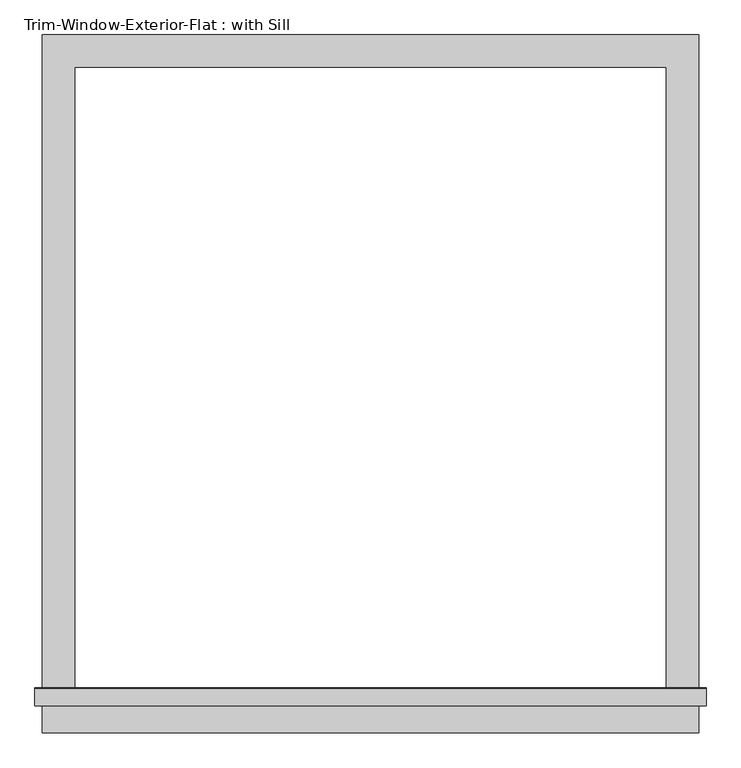
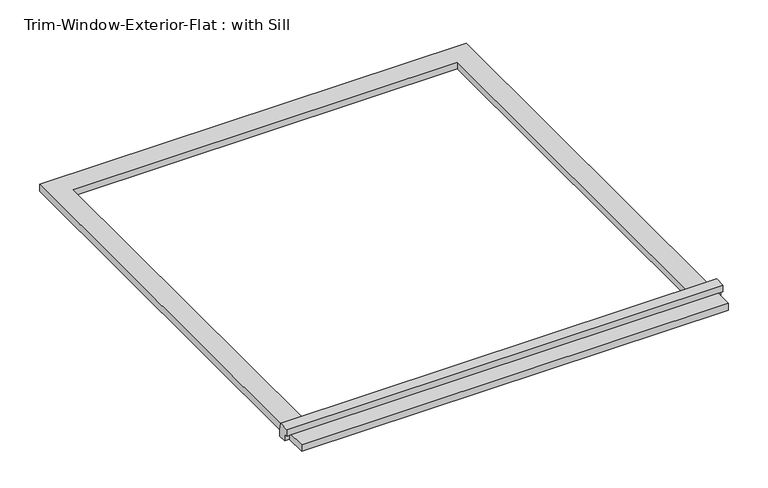
"""IFC4 building model written with IfcOpenShell, lengths in millimetres: proxy geometry, Trim-Window-Exterior-Flat : with Sill."""

import ifcopenshell
import ifcopenshell.guid

model = None  # the IFC model being written
_history = None  # IfcOwnerHistory: only IFC2X3 demands one
_inside = {}  # id of a spatial element -> (the spatial element, [elements in it])
_under = {}  # id of a project, library or spatial element -> (it, [spatial elements below it])
_declared = {}  # id of a project -> (the project, [libraries it declares])
_typed = {}  # id of a type object -> (the type object, [elements of that type])
_made_of = {}  # id of a material, layer set ... -> (it, [elements and type objects made of it])


def new_model(schema):
    """Start an empty IFC model of exactly this schema.

    Asked for "IFC4X3", IfcOpenShell would pick the latest addendum, in which some entities
    have other attributes; the version numbers below select the first issue.
    IFC2X3 requires an IfcOwnerHistory on every rooted entity: one is made here for all.
    """
    global model, _history
    if schema == "IFC4X3":
        model = ifcopenshell.file(schema_version=(4, 3, 0, 0))
    else:
        model = ifcopenshell.file(schema=schema)
    _inside.clear()
    _under.clear()
    _declared.clear()
    _typed.clear()
    _made_of.clear()
    _history = None
    if model.schema == "IFC2X3":
        org = make("IfcOrganization", Name="unknown")
        user = make(
            "IfcPersonAndOrganization",
            ThePerson=make("IfcPerson", FamilyName="unknown"),
            TheOrganization=org,
        )
        app = make(
            "IfcApplication",
            ApplicationDeveloper=org,
            Version="unknown",
            ApplicationFullName="unknown",
            ApplicationIdentifier="unknown",
        )
        _history = make(
            "IfcOwnerHistory",
            OwningUser=user,
            OwningApplication=app,
            ChangeAction="ADDED",
            CreationDate=0,
        )
    return model


def make(cls, **values):
    """One entity of the class cls with the attributes given. An attribute that is None is left unset."""
    return model.create_entity(
        cls, **{name: value for name, value in values.items() if value is not None}
    )


def rooted(cls, **values):
    """An entity with a GlobalId (a new one), such as an element, a storey or a relation."""
    return make(cls, GlobalId=ifcopenshell.guid.new(), OwnerHistory=_history, **values)


def si_unit(unit_type, name, prefix=None):
    """IfcSIUnit, for example si_unit("LENGTHUNIT", "METRE", prefix="MILLI")."""
    return make("IfcSIUnit", UnitType=unit_type, Prefix=prefix, Name=name)


def assignment(units):
    """IfcUnitAssignment: the units of a project."""
    return None if units is None else make("IfcUnitAssignment", Units=units)


def point(xyz):
    """IfcCartesianPoint."""
    return None if xyz is None else make("IfcCartesianPoint", Coordinates=xyz)


def direction(xyz):
    """IfcDirection."""
    return None if xyz is None else make("IfcDirection", DirectionRatios=xyz)


def frame(location, z_axis=None, x_axis=None):
    """IfcAxis2Placement3D, a coordinate frame: its origin and axes. An axis left out is left unset."""
    return make(
        "IfcAxis2Placement3D",
        Location=point(location),
        Axis=direction(z_axis),
        RefDirection=direction(x_axis),
    )


def origin():
    """The frame at (0, 0, 0) with its axes left unset."""
    return frame((0.0, 0.0, 0.0))


def origin_with_axes():
    """The frame at (0, 0, 0) with the z axis (0, 0, 1) and the x axis (1, 0, 0) written out."""
    return frame((0.0, 0.0, 0.0), z_axis=(0.0, 0.0, 1.0), x_axis=(1.0, 0.0, 0.0))


def place(relative_to, where):
    """IfcLocalPlacement: puts the frame where relative to a parent placement (None: the world)."""
    return make(
        "IfcLocalPlacement", PlacementRelTo=relative_to, RelativePlacement=where
    )


def context(
    kind, dimensions, precision=None, world=None, true_north=None, identifier=None
):
    """IfcGeometricRepresentationContext, for example the 3D "Model" context."""
    return make(
        "IfcGeometricRepresentationContext",
        ContextIdentifier=identifier,
        ContextType=kind,
        CoordinateSpaceDimension=dimensions,
        Precision=precision,
        WorldCoordinateSystem=world,
        TrueNorth=true_north,
    )


def project(units=None, contexts=None):
    """IfcProject with its units and contexts."""
    return rooted(
        "IfcProject",
        Name="project",
        RepresentationContexts=contexts,
        UnitsInContext=assignment(units),
    )


def spatial(cls, under=None, at=None, **own):
    """A site, building, storey or space (cls), placed at a placement, below another one or the project."""
    s = rooted(cls, ObjectPlacement=at, **own)
    if under is not None:
        _under.setdefault(under.id(), (under, []))[1].append(s)
    return s


def polyline(points):
    """IfcPolyline through the points."""
    return make("IfcPolyline", Points=[point(p) for p in points])


def outline(outer, holes=None, kind="AREA"):
    """IfcArbitraryClosedProfileDef: a profile drawn as a closed curve; with holes, ...WithVoids."""
    if holes is None:
        return make("IfcArbitraryClosedProfileDef", ProfileType=kind, OuterCurve=outer)
    return make(
        "IfcArbitraryProfileDefWithVoids",
        ProfileType=kind,
        OuterCurve=outer,
        InnerCurves=holes,
    )


def extrude(swept, where, along, depth):
    """IfcExtrudedAreaSolid: the profile swept, set in the frame where, extruded along a direction by depth."""
    return make(
        "IfcExtrudedAreaSolid",
        SweptArea=swept,
        Position=where,
        ExtrudedDirection=direction(along),
        Depth=depth,
    )


def shape(context_of_items, identifier, shape_type, items):
    """IfcShapeRepresentation: the items that make up one representation, for example the "Body"."""
    return make(
        "IfcShapeRepresentation",
        ContextOfItems=context_of_items,
        RepresentationIdentifier=identifier,
        RepresentationType=shape_type,
        Items=items,
    )


def source(mapping_origin, context_of_items, identifier, shape_type, items):
    """IfcRepresentationMap: a shape defined once, which mapped items show again and again."""
    return make(
        "IfcRepresentationMap",
        MappingOrigin=mapping_origin,
        MappedRepresentation=shape(context_of_items, identifier, shape_type, items),
    )


def transform(
    local_origin,
    x_axis=None,
    y_axis=None,
    z_axis=None,
    scale=None,
    scale2=None,
    scale3=None,
    uniform=True,
):
    """IfcCartesianTransformationOperator3D, or its non-uniform kind. x_axis, y_axis, z_axis: its Axis1, 2, 3."""
    if uniform:
        return make(
            "IfcCartesianTransformationOperator3D",
            Axis1=direction(x_axis),
            Axis2=direction(y_axis),
            LocalOrigin=point(local_origin),
            Scale=scale,
            Axis3=direction(z_axis),
        )
    return make(
        "IfcCartesianTransformationOperator3DnonUniform",
        Axis1=direction(x_axis),
        Axis2=direction(y_axis),
        LocalOrigin=point(local_origin),
        Scale=scale,
        Axis3=direction(z_axis),
        Scale2=scale2,
        Scale3=scale3,
    )


def mapped(mapping_source, mapping_target):
    """IfcMappedItem: shows the shape of a source again, moved by a transform."""
    return make(
        "IfcMappedItem", MappingSource=mapping_source, MappingTarget=mapping_target
    )


def made_of(thing, what):
    """Note that an element or type object is made of a material, layer set ...; save() writes the relation."""
    if what is not None:
        _made_of.setdefault(what.id(), (what, []))[1].append(thing)
    return thing


def element(
    cls,
    number,
    at=None,
    inside=None,
    cuts=None,
    type_object=None,
    material=None,
    context=None,
    identifier="Body",
    shape_type=None,
    held_by="IfcProductDefinitionShape",
    body=None,
    shapes=None,
    **own,
):
    """One element of the class cls, such as IfcWall. Its Tag is "e" and its number.

    at: its placement. inside: the storey or other place that contains it. cuts: it is an
    opening in that element (IfcRelVoidsElement). A single representation is given by context,
    identifier, shape_type and body (its items); several are given by shapes. held_by: the class
    of the entity that holds the representations. save() writes the other relations.
    """
    e = rooted(cls, Tag="e%d" % number, ObjectPlacement=at, **own)
    if body is not None:
        shapes = [shape(context, identifier, shape_type, body)]
    if shapes is not None:
        e.Representation = make(held_by, Representations=shapes)
    if inside is not None:
        _inside.setdefault(inside.id(), (inside, []))[1].append(e)
    if cuts is not None:
        rooted(
            "IfcRelVoidsElement", RelatingBuildingElement=cuts, RelatedOpeningElement=e
        )
    if type_object is not None:
        _typed.setdefault(type_object.id(), (type_object, []))[1].append(e)
    return made_of(e, material)


def aggregate(whole, parts):
    """IfcRelAggregates: a whole, such as a stair, and the parts it consists of."""
    return rooted("IfcRelAggregates", RelatingObject=whole, RelatedObjects=parts)


def save(model, path):
    """Write the relations noted so far, then the file.

    IfcRelAggregates (storeys below a building ...), IfcRelContainedInSpatialStructure (elements
    in a storey), IfcRelDefinesByType, IfcRelAssociatesMaterial and IfcRelDeclares: one each for
    every whole, place, type object, material and project.
    """
    for whole, parts in _under.values():
        aggregate(whole, parts)
    for where, things in _inside.values():
        rooted(
            "IfcRelContainedInSpatialStructure",
            RelatedElements=things,
            RelatingStructure=where,
        )
    for kind, things in _typed.values():
        rooted("IfcRelDefinesByType", RelatedObjects=things, RelatingType=kind)
    for what, things in _made_of.values():
        rooted("IfcRelAssociatesMaterial", RelatedObjects=things, RelatingMaterial=what)
    for by, libraries in _declared.values():
        rooted("IfcRelDeclares", RelatingContext=by, RelatedDefinitions=libraries)
    model.write(path)


def trim_window_exterior_flat_with_sill_d43e16eb(model_context):
    return source(origin(), model_context, "Body", "SweptSolid", [
        extrude(outline(polyline([(577.85, -1114.3823709), (577.85, -1171.5323709), (-577.85, -1171.5323709), (-577.85, -1114.3823709), (577.85, -1114.3823709)])), origin_with_axes(), (0.0, 0.0, 1.0), 19.05),
        extrude(outline(polyline([(-1123.95, 38.1), (-1094.6580645, 38.1), (-1092.2, 19.05), (-1092.2, 0.0), (-1114.3823709, 0.0), (-1114.3823709, 19.05), (-1123.95, 19.05), (-1123.95, 38.1)])), frame((-590.55, 0.0, 0.0), z_axis=(1.0, 0.0, 0.0), x_axis=(0.0, 1.0, 0.0)), (0.0, 0.0, 1.0), 1181.1),
        extrude(outline(polyline([(-577.85, 57.15), (577.85, 57.15), (577.85, -1092.2), (520.7, -1092.2), (520.7, 0.0), (-520.7, 0.0), (-520.7, -1092.2), (-577.85, -1092.2), (-577.85, 57.15)])), origin_with_axes(), (0.0, 0.0, 1.0), 19.05),
    ])


if __name__ == "__main__":
    model = new_model("IFC4")
    model_context = context("Model", 3, world=origin())
    ifc_project = project(units=[si_unit("LENGTHUNIT", "METRE", prefix="MILLI")], contexts=[model_context])
    site = spatial("IfcSite", under=ifc_project)
    building = spatial("IfcBuilding", under=site)
    placement = place(None, origin())
    trim_window_exterior_flat_with_sill_shape = trim_window_exterior_flat_with_sill_d43e16eb(model_context)
    element("IfcBuildingElementProxy", 1, Name="Trim-Window-Exterior-Flat : with Sill", ObjectType="Trim-Window-Exterior-Flat : with Sill", at=placement, inside=building, context=model_context, shape_type="MappedRepresentation", body=[
        mapped(trim_window_exterior_flat_with_sill_shape, transform((0.0, 0.0, 0.0), x_axis=(1.0, 0.0, 0.0), y_axis=(0.0, 1.0, 0.0), z_axis=(0.0, 0.0, 1.0))),
    ])
    save(model, "model.ifc")

# Revit data of these elements
# Type "Trim-Window-Exterior-Flat : with Sill"
#   Trim Width = 0' - 2 1/4"
#   Trim Thickness_Picture Frame = 0' - 1 1/4"
#   Trim Thickness_with Sill = 0' - 0 3/4"
#   Sill Thickness = 0' - 1 1/4"
#   Opening Width [instance default] = 2' - 0"
#   Opening Height [instance default] = 3' - 0"
#   Default Elevation = 4' - 0"
#   Sill = yes
#   Picture Frame = no
#   Trim Material [instance default] = none
# Element 1 (IfcBuildingElementProxy, "Trim-Window-Exterior-Flat : with Sill")
#   Opening Width = 3' - 5"
#   Opening Height = 3' - 7"
#   Trim Material = 1X WOOD COMPOSITE TRIM
#   Materials on its faces: "1X WOOD COMPOSITE TRIM"
# Materials
#   "1X WOOD COMPOSITE TRIM": class "Generic", colour RGB 88 61 61, transparency 0, Cost = 0
